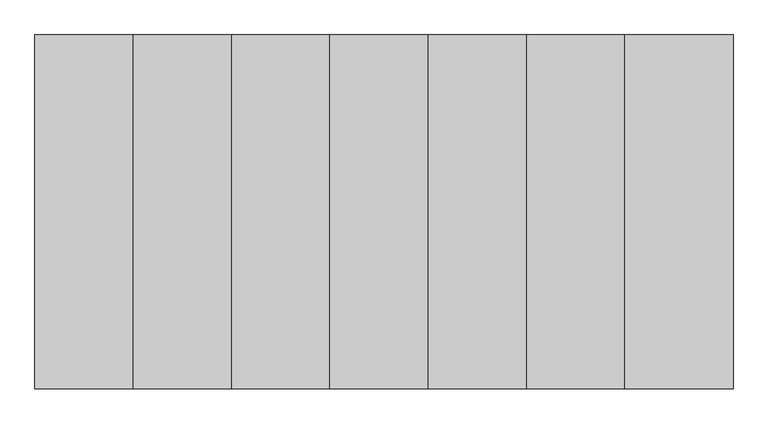
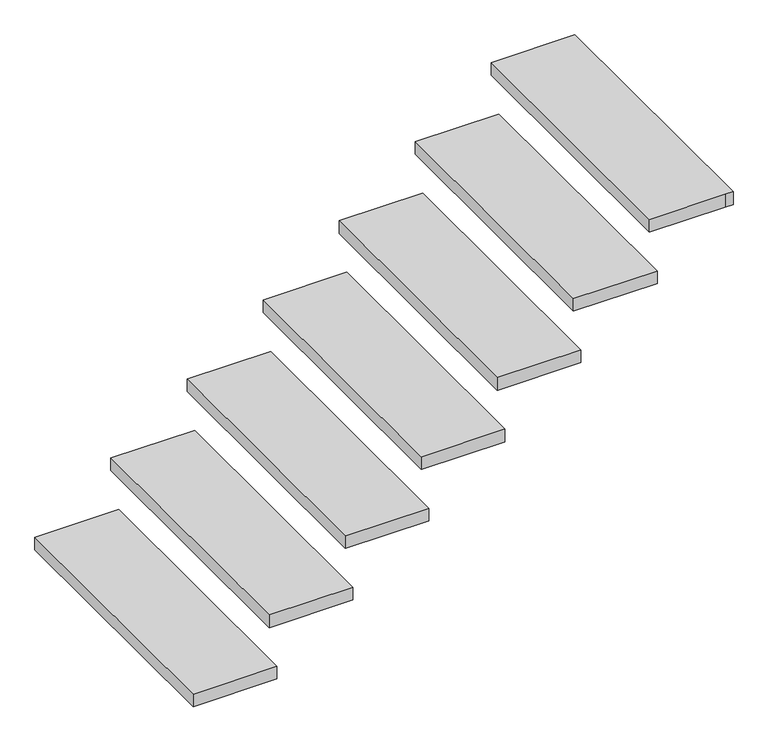
"""IFC4 building model written with IfcOpenShell, lengths in millimetres: stair flight geometry."""

import ifcopenshell
import ifcopenshell.guid

model = None  # the IFC model being written
_history = None  # IfcOwnerHistory: only IFC2X3 demands one
_inside = {}  # id of a spatial element -> (the spatial element, [elements in it])
_under = {}  # id of a project, library or spatial element -> (it, [spatial elements below it])
_declared = {}  # id of a project -> (the project, [libraries it declares])
_typed = {}  # id of a type object -> (the type object, [elements of that type])
_made_of = {}  # id of a material, layer set ... -> (it, [elements and type objects made of it])


def new_model(schema):
    """Start an empty IFC model of exactly this schema.

    Asked for "IFC4X3", IfcOpenShell would pick the latest addendum, in which some entities
    have other attributes; the version numbers below select the first issue.
    IFC2X3 requires an IfcOwnerHistory on every rooted entity: one is made here for all.
    """
    global model, _history
    if schema == "IFC4X3":
        model = ifcopenshell.file(schema_version=(4, 3, 0, 0))
    else:
        model = ifcopenshell.file(schema=schema)
    _inside.clear()
    _under.clear()
    _declared.clear()
    _typed.clear()
    _made_of.clear()
    _history = None
    if model.schema == "IFC2X3":
        org = make("IfcOrganization", Name="unknown")
        user = make(
            "IfcPersonAndOrganization",
            ThePerson=make("IfcPerson", FamilyName="unknown"),
            TheOrganization=org,
        )
        app = make(
            "IfcApplication",
            ApplicationDeveloper=org,
            Version="unknown",
            ApplicationFullName="unknown",
            ApplicationIdentifier="unknown",
        )
        _history = make(
            "IfcOwnerHistory",
            OwningUser=user,
            OwningApplication=app,
            ChangeAction="ADDED",
            CreationDate=0,
        )
    return model


def make(cls, **values):
    """One entity of the class cls with the attributes given. An attribute that is None is left unset."""
    return model.create_entity(
        cls, **{name: value for name, value in values.items() if value is not None}
    )


def rooted(cls, **values):
    """An entity with a GlobalId (a new one), such as an element, a storey or a relation."""
    return make(cls, GlobalId=ifcopenshell.guid.new(), OwnerHistory=_history, **values)


def si_unit(unit_type, name, prefix=None):
    """IfcSIUnit, for example si_unit("LENGTHUNIT", "METRE", prefix="MILLI")."""
    return make("IfcSIUnit", UnitType=unit_type, Prefix=prefix, Name=name)


def assignment(units):
    """IfcUnitAssignment: the units of a project."""
    return None if units is None else make("IfcUnitAssignment", Units=units)


def point(xyz):
    """IfcCartesianPoint."""
    return None if xyz is None else make("IfcCartesianPoint", Coordinates=xyz)


def direction(xyz):
    """IfcDirection."""
    return None if xyz is None else make("IfcDirection", DirectionRatios=xyz)


def frame(location, z_axis=None, x_axis=None):
    """IfcAxis2Placement3D, a coordinate frame: its origin and axes. An axis left out is left unset."""
    return make(
        "IfcAxis2Placement3D",
        Location=point(location),
        Axis=direction(z_axis),
        RefDirection=direction(x_axis),
    )


def origin():
    """The frame at (0, 0, 0) with its axes left unset."""
    return frame((0.0, 0.0, 0.0))


def place(relative_to, where):
    """IfcLocalPlacement: puts the frame where relative to a parent placement (None: the world)."""
    return make(
        "IfcLocalPlacement", PlacementRelTo=relative_to, RelativePlacement=where
    )


def context(
    kind, dimensions, precision=None, world=None, true_north=None, identifier=None
):
    """IfcGeometricRepresentationContext, for example the 3D "Model" context."""
    return make(
        "IfcGeometricRepresentationContext",
        ContextIdentifier=identifier,
        ContextType=kind,
        CoordinateSpaceDimension=dimensions,
        Precision=precision,
        WorldCoordinateSystem=world,
        TrueNorth=true_north,
    )


def project(units=None, contexts=None):
    """IfcProject with its units and contexts."""
    return rooted(
        "IfcProject",
        Name="project",
        RepresentationContexts=contexts,
        UnitsInContext=assignment(units),
    )


def spatial(cls, under=None, at=None, **own):
    """A site, building, storey or space (cls), placed at a placement, below another one or the project."""
    s = rooted(cls, ObjectPlacement=at, **own)
    if under is not None:
        _under.setdefault(under.id(), (under, []))[1].append(s)
    return s


def polyline(points):
    """IfcPolyline through the points."""
    return make("IfcPolyline", Points=[point(p) for p in points])


def outline(outer, holes=None, kind="AREA"):
    """IfcArbitraryClosedProfileDef: a profile drawn as a closed curve; with holes, ...WithVoids."""
    if holes is None:
        return make("IfcArbitraryClosedProfileDef", ProfileType=kind, OuterCurve=outer)
    return make(
        "IfcArbitraryProfileDefWithVoids",
        ProfileType=kind,
        OuterCurve=outer,
        InnerCurves=holes,
    )


def extrude(swept, where, along, depth):
    """IfcExtrudedAreaSolid: the profile swept, set in the frame where, extruded along a direction by depth."""
    return make(
        "IfcExtrudedAreaSolid",
        SweptArea=swept,
        Position=where,
        ExtrudedDirection=direction(along),
        Depth=depth,
    )


def shape(context_of_items, identifier, shape_type, items):
    """IfcShapeRepresentation: the items that make up one representation, for example the "Body"."""
    return make(
        "IfcShapeRepresentation",
        ContextOfItems=context_of_items,
        RepresentationIdentifier=identifier,
        RepresentationType=shape_type,
        Items=items,
    )


def source(mapping_origin, context_of_items, identifier, shape_type, items):
    """IfcRepresentationMap: a shape defined once, which mapped items show again and again."""
    return make(
        "IfcRepresentationMap",
        MappingOrigin=mapping_origin,
        MappedRepresentation=shape(context_of_items, identifier, shape_type, items),
    )


def transform(
    local_origin,
    x_axis=None,
    y_axis=None,
    z_axis=None,
    scale=None,
    scale2=None,
    scale3=None,
    uniform=True,
):
    """IfcCartesianTransformationOperator3D, or its non-uniform kind. x_axis, y_axis, z_axis: its Axis1, 2, 3."""
    if uniform:
        return make(
            "IfcCartesianTransformationOperator3D",
            Axis1=direction(x_axis),
            Axis2=direction(y_axis),
            LocalOrigin=point(local_origin),
            Scale=scale,
            Axis3=direction(z_axis),
        )
    return make(
        "IfcCartesianTransformationOperator3DnonUniform",
        Axis1=direction(x_axis),
        Axis2=direction(y_axis),
        LocalOrigin=point(local_origin),
        Scale=scale,
        Axis3=direction(z_axis),
        Scale2=scale2,
        Scale3=scale3,
    )


def mapped(mapping_source, mapping_target):
    """IfcMappedItem: shows the shape of a source again, moved by a transform."""
    return make(
        "IfcMappedItem", MappingSource=mapping_source, MappingTarget=mapping_target
    )


def made_of(thing, what):
    """Note that an element or type object is made of a material, layer set ...; save() writes the relation."""
    if what is not None:
        _made_of.setdefault(what.id(), (what, []))[1].append(thing)
    return thing


def element(
    cls,
    number,
    at=None,
    inside=None,
    cuts=None,
    type_object=None,
    material=None,
    context=None,
    identifier="Body",
    shape_type=None,
    held_by="IfcProductDefinitionShape",
    body=None,
    shapes=None,
    **own,
):
    """One element of the class cls, such as IfcWall. Its Tag is "e" and its number.

    at: its placement. inside: the storey or other place that contains it. cuts: it is an
    opening in that element (IfcRelVoidsElement). A single representation is given by context,
    identifier, shape_type and body (its items); several are given by shapes. held_by: the class
    of the entity that holds the representations. save() writes the other relations.
    """
    e = rooted(cls, Tag="e%d" % number, ObjectPlacement=at, **own)
    if body is not None:
        shapes = [shape(context, identifier, shape_type, body)]
    if shapes is not None:
        e.Representation = make(held_by, Representations=shapes)
    if inside is not None:
        _inside.setdefault(inside.id(), (inside, []))[1].append(e)
    if cuts is not None:
        rooted(
            "IfcRelVoidsElement", RelatingBuildingElement=cuts, RelatedOpeningElement=e
        )
    if type_object is not None:
        _typed.setdefault(type_object.id(), (type_object, []))[1].append(e)
    return made_of(e, material)


def aggregate(whole, parts):
    """IfcRelAggregates: a whole, such as a stair, and the parts it consists of."""
    return rooted("IfcRelAggregates", RelatingObject=whole, RelatedObjects=parts)


def save(model, path):
    """Write the relations noted so far, then the file.

    IfcRelAggregates (storeys below a building ...), IfcRelContainedInSpatialStructure (elements
    in a storey), IfcRelDefinesByType, IfcRelAssociatesMaterial and IfcRelDeclares: one each for
    every whole, place, type object, material and project.
    """
    for whole, parts in _under.values():
        aggregate(whole, parts)
    for where, things in _inside.values():
        rooted(
            "IfcRelContainedInSpatialStructure",
            RelatedElements=things,
            RelatingStructure=where,
        )
    for kind, things in _typed.values():
        rooted("IfcRelDefinesByType", RelatedObjects=things, RelatingType=kind)
    for what, things in _made_of.values():
        rooted("IfcRelAssociatesMaterial", RelatedObjects=things, RelatingMaterial=what)
    for by, libraries in _declared.values():
        rooted("IfcRelDeclares", RelatingContext=by, RelatedDefinitions=libraries)
    model.write(path)


def stair_flight_2204dae2(model_context):
    return source(origin(), model_context, "Body", "SweptSolid", [
        extrude(outline(polyline([(-17502.6481446, -4273.6871906), (-17502.6481446, -5188.0871906), (-17782.0481446, -5188.0871906), (-17782.0481446, -4273.6871906), (-17502.6481446, -4273.6871906)])), frame((0.0, 0.0, 146.05), z_axis=(0.0, 0.0, 1.0), x_axis=(1.0, 0.0, 0.0)), (0.0, 0.0, 1.0), 44.45),
        extrude(outline(polyline([(-15978.6481446, -4273.6871906), (-15978.6481446, -5188.0871906), (-16004.0481446, -5188.0871906), (-16258.0481446, -5188.0871906), (-16258.0481446, -4273.6871906), (-15978.6481446, -4273.6871906)])), frame((0.0, 0.0, 1289.05), z_axis=(0.0, 0.0, 1.0), x_axis=(1.0, 0.0, 0.0)), (0.0, 0.0, 1.0), 44.45),
        extrude(outline(polyline([(-17248.6481446, -4273.6871906), (-17248.6481446, -5188.0871906), (-17528.0481446, -5188.0871906), (-17528.0481446, -4273.6871906), (-17248.6481446, -4273.6871906)])), frame((0.0, 0.0, 336.55), z_axis=(0.0, 0.0, 1.0), x_axis=(1.0, 0.0, 0.0)), (0.0, 0.0, 1.0), 44.45),
        extrude(outline(polyline([(-16994.6481446, -4273.6871906), (-16994.6481446, -5188.0871906), (-17274.0481446, -5188.0871906), (-17274.0481446, -4273.6871906), (-16994.6481446, -4273.6871906)])), frame((0.0, 0.0, 527.05), z_axis=(0.0, 0.0, 1.0), x_axis=(1.0, 0.0, 0.0)), (0.0, 0.0, 1.0), 44.45),
        extrude(outline(polyline([(-16740.6481446, -4273.6871906), (-16740.6481446, -5188.0871906), (-17020.0481446, -5188.0871906), (-17020.0481446, -4273.6871906), (-16740.6481446, -4273.6871906)])), frame((0.0, 0.0, 717.55), z_axis=(0.0, 0.0, 1.0), x_axis=(1.0, 0.0, 0.0)), (0.0, 0.0, 1.0), 44.45),
        extrude(outline(polyline([(-16486.6481446, -4273.6871906), (-16486.6481446, -5188.0871906), (-16766.0481446, -5188.0871906), (-16766.0481446, -4273.6871906), (-16486.6481446, -4273.6871906)])), frame((0.0, 0.0, 908.05), z_axis=(0.0, 0.0, 1.0), x_axis=(1.0, 0.0, 0.0)), (0.0, 0.0, 1.0), 44.45),
        extrude(outline(polyline([(-16232.6481446, -4273.6871906), (-16232.6481446, -5188.0871906), (-16512.0481446, -5188.0871906), (-16512.0481446, -4273.6871906), (-16232.6481446, -4273.6871906)])), frame((0.0, 0.0, 1098.55), z_axis=(0.0, 0.0, 1.0), x_axis=(1.0, 0.0, 0.0)), (0.0, 0.0, 1.0), 44.45),
    ])


if __name__ == "__main__":
    model = new_model("IFC4")
    model_context = context("Model", 3, world=origin())
    ifc_project = project(units=[si_unit("LENGTHUNIT", "METRE", prefix="MILLI")], contexts=[model_context])
    site = spatial("IfcSite", under=ifc_project)
    building = spatial("IfcBuilding", under=site)
    placement = place(None, origin())
    stair_flight_shape = stair_flight_2204dae2(model_context)
    element("IfcStairFlight", 1, at=placement, inside=building, context=model_context, shape_type="MappedRepresentation", body=[
        mapped(stair_flight_shape, transform((0.0, 0.0, 0.0), x_axis=(1.0, 0.0, 0.0), y_axis=(0.0, 1.0, 0.0), z_axis=(0.0, 0.0, 1.0))),
    ])
    save(model, "model.ifc")

# Revit data of these elements
# Element 1 (IfcStairFlight)
#   Materials on its faces: "Wood - Flooring"
# Materials
#   "Wood - Flooring": class "Unassigned", colour RGB 216 169 114, transparency 0
